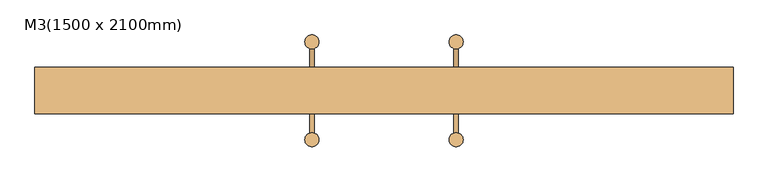
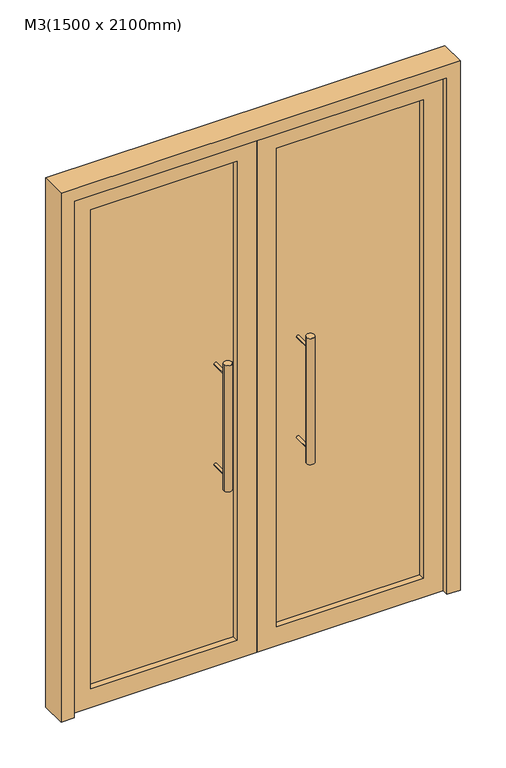
"""IFC4 building model written with IfcOpenShell, lengths in millimetres: door geometry, 双面嵌板玻璃门 : M3(1500 x 2100mm)."""

from ifc_helpers import new_model, si_unit, point, frame, frame_2d, origin, place, context, project, spatial, polyline, circle_curve, trimmed, segment, composite_curve, outline, extrude, source, transform, mapped, element, save


def m3_1500_x_2100mm_b0fe12bd(model_context):
    return source(origin(), model_context, "Body", "SweptSolid", [
        extrude(outline(composite_curve([segment(trimmed(circle_curve(frame_2d((155.0, 105.0)), 15.0), [point((140.0, 105.0))], [point((170.0, 105.0))], False, "CARTESIAN"), True, "CONTINUOUS"), segment(trimmed(circle_curve(frame_2d((155.0, 105.0)), 15.0), [point((170.0, 105.0))], [point((140.0, 105.0))], False, "CARTESIAN"), True, "CONTINUOUS")], self_intersect=False)), frame((0.0, 0.0, 750.0), z_axis=(0.0, 0.0, 1.0), x_axis=(1.0, 0.0, 0.0)), (0.0, 0.0, 1.0), 500.0),
        extrude(outline(composite_curve([segment(trimmed(circle_curve(frame_2d((1200.0, 155.0)), 5.0), [point((1200.0, 150.0))], [point((1200.0, 160.0))], False, "CARTESIAN"), True, "CONTINUOUS"), segment(trimmed(circle_curve(frame_2d((1200.0, 155.0)), 5.0), [point((1200.0, 160.0))], [point((1200.0, 150.0))], False, "CARTESIAN"), True, "CONTINUOUS")], self_intersect=False)), frame((0.0, 25.0, 0.0), z_axis=(0.0, 1.0, 0.0), x_axis=(0.0, 0.0, 1.0)), (0.0, 0.0, 1.0), 80.0),
        extrude(outline(composite_curve([segment(trimmed(circle_curve(frame_2d((800.0, 155.0)), 5.0), [point((800.0, 150.0))], [point((800.0, 160.0))], False, "CARTESIAN"), True, "CONTINUOUS"), segment(trimmed(circle_curve(frame_2d((800.0, 155.0)), 5.0), [point((800.0, 160.0))], [point((800.0, 150.0))], False, "CARTESIAN"), True, "CONTINUOUS")], self_intersect=False)), frame((0.0, 25.0, 0.0), z_axis=(0.0, 1.0, 0.0), x_axis=(0.0, 0.0, 1.0)), (0.0, 0.0, 1.0), 80.0),
        extrude(outline(composite_curve([segment(trimmed(circle_curve(frame_2d((1200.0, 155.0)), 5.0), [point((1200.0, 150.0))], [point((1200.0, 160.0))], False, "CARTESIAN"), True, "CONTINUOUS"), segment(trimmed(circle_curve(frame_2d((1200.0, 155.0)), 5.0), [point((1200.0, 160.0))], [point((1200.0, 150.0))], False, "CARTESIAN"), True, "CONTINUOUS")], self_intersect=False)), frame((0.0, -105.0, 0.0), z_axis=(0.0, 1.0, 0.0), x_axis=(0.0, 0.0, 1.0)), (0.0, 0.0, 1.0), 80.0),
        extrude(outline(composite_curve([segment(trimmed(circle_curve(frame_2d((800.0, 155.0)), 5.0), [point((800.0, 150.0))], [point((800.0, 160.0))], False, "CARTESIAN"), True, "CONTINUOUS"), segment(trimmed(circle_curve(frame_2d((800.0, 155.0)), 5.0), [point((800.0, 160.0))], [point((800.0, 150.0))], False, "CARTESIAN"), True, "CONTINUOUS")], self_intersect=False)), frame((0.0, -105.0, 0.0), z_axis=(0.0, 1.0, 0.0), x_axis=(0.0, 0.0, 1.0)), (0.0, 0.0, 1.0), 80.0),
        extrude(outline(composite_curve([segment(trimmed(circle_curve(frame_2d((155.0, -105.0)), 15.0), [point((140.0, -105.0))], [point((170.0, -105.0))], False, "CARTESIAN"), True, "CONTINUOUS"), segment(trimmed(circle_curve(frame_2d((155.0, -105.0)), 15.0), [point((170.0, -105.0))], [point((140.0, -105.0))], False, "CARTESIAN"), True, "CONTINUOUS")], self_intersect=False)), frame((0.0, 0.0, 750.0), z_axis=(0.0, 0.0, 1.0), x_axis=(1.0, 0.0, 0.0)), (0.0, 0.0, 1.0), 500.0),
        extrude(outline(composite_curve([segment(trimmed(circle_curve(frame_2d((-155.0, 105.0)), 15.0), [point((-170.0, 105.0))], [point((-140.0, 105.0))], False, "CARTESIAN"), True, "CONTINUOUS"), segment(trimmed(circle_curve(frame_2d((-155.0, 105.0)), 15.0), [point((-140.0, 105.0))], [point((-170.0, 105.0))], False, "CARTESIAN"), True, "CONTINUOUS")], self_intersect=False)), frame((0.0, 0.0, 750.0), z_axis=(0.0, 0.0, 1.0), x_axis=(1.0, 0.0, 0.0)), (0.0, 0.0, 1.0), 500.0),
        extrude(outline(composite_curve([segment(trimmed(circle_curve(frame_2d((1200.0, -155.0)), 5.0), [point((1200.0, -160.0))], [point((1200.0, -150.0))], False, "CARTESIAN"), True, "CONTINUOUS"), segment(trimmed(circle_curve(frame_2d((1200.0, -155.0)), 5.0), [point((1200.0, -150.0))], [point((1200.0, -160.0))], False, "CARTESIAN"), True, "CONTINUOUS")], self_intersect=False)), frame((0.0, 25.0, 0.0), z_axis=(0.0, 1.0, 0.0), x_axis=(0.0, 0.0, 1.0)), (0.0, 0.0, 1.0), 80.0),
        extrude(outline(composite_curve([segment(trimmed(circle_curve(frame_2d((800.0, -155.0)), 5.0), [point((800.0, -160.0))], [point((800.0, -150.0))], False, "CARTESIAN"), True, "CONTINUOUS"), segment(trimmed(circle_curve(frame_2d((800.0, -155.0)), 5.0), [point((800.0, -150.0))], [point((800.0, -160.0))], False, "CARTESIAN"), True, "CONTINUOUS")], self_intersect=False)), frame((0.0, 25.0, 0.0), z_axis=(0.0, 1.0, 0.0), x_axis=(0.0, 0.0, 1.0)), (0.0, 0.0, 1.0), 80.0),
        extrude(outline(composite_curve([segment(trimmed(circle_curve(frame_2d((1200.0, -155.0)), 5.0), [point((1200.0, -160.0))], [point((1200.0, -150.0))], False, "CARTESIAN"), True, "CONTINUOUS"), segment(trimmed(circle_curve(frame_2d((1200.0, -155.0)), 5.0), [point((1200.0, -150.0))], [point((1200.0, -160.0))], False, "CARTESIAN"), True, "CONTINUOUS")], self_intersect=False)), frame((0.0, -105.0, 0.0), z_axis=(0.0, 1.0, 0.0), x_axis=(0.0, 0.0, 1.0)), (0.0, 0.0, 1.0), 80.0),
        extrude(outline(composite_curve([segment(trimmed(circle_curve(frame_2d((800.0, -155.0)), 5.0), [point((800.0, -160.0))], [point((800.0, -150.0))], False, "CARTESIAN"), True, "CONTINUOUS"), segment(trimmed(circle_curve(frame_2d((800.0, -155.0)), 5.0), [point((800.0, -150.0))], [point((800.0, -160.0))], False, "CARTESIAN"), True, "CONTINUOUS")], self_intersect=False)), frame((0.0, -105.0, 0.0), z_axis=(0.0, 1.0, 0.0), x_axis=(0.0, 0.0, 1.0)), (0.0, 0.0, 1.0), 80.0),
        extrude(outline(composite_curve([segment(trimmed(circle_curve(frame_2d((-155.0, -105.0)), 15.0), [point((-170.0, -105.0))], [point((-140.0, -105.0))], False, "CARTESIAN"), True, "CONTINUOUS"), segment(trimmed(circle_curve(frame_2d((-155.0, -105.0)), 15.0), [point((-140.0, -105.0))], [point((-170.0, -105.0))], False, "CARTESIAN"), True, "CONTINUOUS")], self_intersect=False)), frame((0.0, 0.0, 750.0), z_axis=(0.0, 0.0, 1.0), x_axis=(1.0, 0.0, 0.0)), (0.0, 0.0, 1.0), 500.0),
        extrude(outline(polyline([(75.0, 2.0), (625.0, 2.0), (625.0, -2.0), (75.0, -2.0), (75.0, 2.0)])), frame((0.0, 0.0, 75.0), z_axis=(0.0, 0.0, 1.0), x_axis=(1.0, 0.0, 0.0)), (0.0, 0.0, 1.0), 1900.0),
        extrude(outline(polyline([(-625.0, 2.0), (-75.0, 2.0), (-75.0, -2.0), (-625.0, -2.0), (-625.0, 2.0)])), frame((0.0, 0.0, 75.0), z_axis=(0.0, 0.0, 1.0), x_axis=(1.0, 0.0, 0.0)), (0.0, 0.0, 1.0), 1900.0),
        extrude(outline(polyline([(2050.0, 0.0), (2050.0, -700.0), (0.0, -700.0), (0.0, 0.0), (2050.0, 0.0)]), holes=[polyline([(1975.0, -625.0), (1975.0, -75.0), (75.0, -75.0), (75.0, -625.0), (1975.0, -625.0)])]), frame((0.0, -25.0, 0.0), z_axis=(0.0, 1.0, 0.0), x_axis=(0.0, 0.0, 1.0)), (0.0, 0.0, 1.0), 50.0),
        extrude(outline(polyline([(2050.0, 0.0), (0.0, 0.0), (0.0, 700.0), (2050.0, 700.0), (2050.0, 0.0)]), holes=[polyline([(1975.0, 625.0), (75.0, 625.0), (75.0, 75.0), (1975.0, 75.0), (1975.0, 625.0)])]), frame((0.0, -25.0, 0.0), z_axis=(0.0, 1.0, 0.0), x_axis=(0.0, 0.0, 1.0)), (0.0, 0.0, 1.0), 50.0),
        extrude(outline(polyline([(2100.0, 750.0), (2100.0, -750.0), (0.0, -750.0), (0.0, -700.0), (2050.0, -700.0), (2050.0, 700.0), (0.0, 700.0), (0.0, 750.0), (2100.0, 750.0)])), frame((0.0, -50.0, 0.0), z_axis=(0.0, 1.0, 0.0), x_axis=(0.0, 0.0, 1.0)), (0.0, 0.0, 1.0), 100.0),
    ])


if __name__ == "__main__":
    model = new_model("IFC4")
    model_context = context("Model", 3, world=origin())
    ifc_project = project(units=[si_unit("LENGTHUNIT", "METRE", prefix="MILLI")], contexts=[model_context])
    site = spatial("IfcSite", under=ifc_project)
    building = spatial("IfcBuilding", under=site)
    placement = place(None, origin())
    m3_1500_x_2100mm_shape = m3_1500_x_2100mm_b0fe12bd(model_context)
    element("IfcDoor", 1, ObjectType="双面嵌板玻璃门 : M3(1500 x 2100mm)", at=placement, inside=building, context=model_context, shape_type="MappedRepresentation", body=[
        mapped(m3_1500_x_2100mm_shape, transform((0.0, 0.0, 0.0), x_axis=(1.0, 0.0, 0.0), y_axis=(0.0, 1.0, 0.0), z_axis=(0.0, 0.0, 1.0))),
    ])
    save(model, "model.ifc")

# Revit data of these elements
# Type "双面嵌板玻璃门 : M3(1500 x 2100mm)"
#   Type Mark = "M833"
#   Construction Type Id = "GSP4R"
#   Analytic Construction = "1/8 英寸 Pilkington 单层玻璃"
#   Visual Light Transmittance = 0.9
#   Thickness = 50 mm
#   Solar Heat Gain Coefficient = 0.78
#   Rough Width = 1800 mm
#   Rough Height = 2400 mm
#   W = 750 mm
#   Heat Transfer Coefficient (U) = 3.6886 W/(m²·K)
#   门嵌板框架宽度 = 75 mm
#   门嵌板框架厚度 = 50 mm
#   Height = 2100 mm
#   Width = 1500 mm
#   框架宽度 = 50 mm
#   框架厚度 = 100 mm
#   把手材质 = none
#   玻璃 = none
#   框架材质 = none
#   门嵌板框架材质 = none
#   Type Comments = ""
#   Function = (empty or 0)
#   Wall Closure = (empty or 0)
#   Construction Type = (empty or 0)
# Element 1 (IfcDoor, "双面嵌板玻璃门 : M3(1500 x 2100mm)")
#   Materials on its faces: "玻璃"
# Materials
#   "玻璃": class "玻璃", colour RGB 0 128 192, transparency 0.9, Description = "钠钙玻璃", Cost = 0
